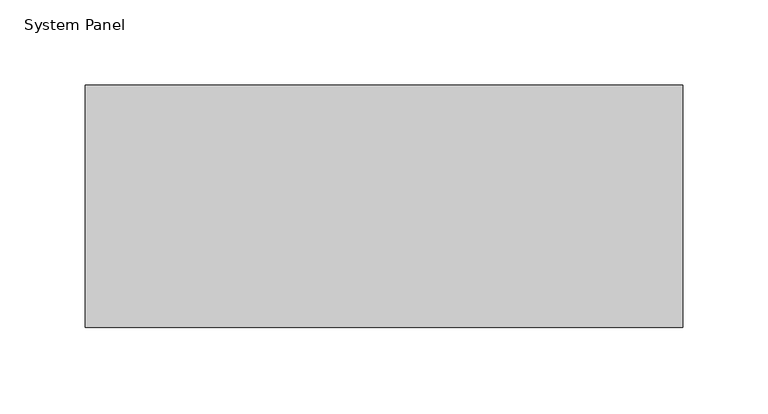
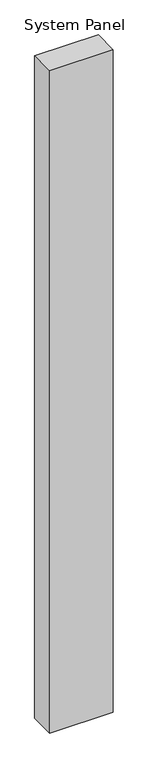
"""IFC4 building model written with IfcOpenShell, lengths in millimetres: plate geometry, System Panel : NLRS_21_CWP_hsb-vulling minerale wol 142 _gen_rsf."""

from ifc_helpers import new_model, si_unit, origin, origin_with_axes, place, context, project, spatial, polyline, outline, extrude, source, transform, mapped, element, save


def system_panel_cc2e8257(model_context):
    return source(origin(), model_context, "Body", "SweptSolid", [
        extrude(outline(polyline([(175.0000002, -71.0), (-175.0000002, -71.0), (-175.0000002, 71.0), (175.0000002, 71.0), (175.0000002, -71.0)])), origin_with_axes(), (0.0, 0.0, 1.0), 3849.0),
    ])


if __name__ == "__main__":
    model = new_model("IFC4")
    model_context = context("Model", 3, world=origin())
    ifc_project = project(units=[si_unit("LENGTHUNIT", "METRE", prefix="MILLI")], contexts=[model_context])
    site = spatial("IfcSite", under=ifc_project)
    building = spatial("IfcBuilding", under=site)
    placement = place(None, origin())
    system_panel_shape = system_panel_cc2e8257(model_context)
    element("IfcPlate", 1, ObjectType="System Panel : NLRS_21_CWP_hsb-vulling minerale wol 142 _gen_rsf", at=placement, inside=building, context=model_context, shape_type="MappedRepresentation", body=[
        mapped(system_panel_shape, transform((0.0, 0.0, 0.0), x_axis=(1.0, 0.0, 0.0), y_axis=(0.0, 1.0, 0.0), z_axis=(0.0, 0.0, 1.0))),
    ])
    save(model, "model.ifc")

# Revit data of these elements
# Type "System Panel : NLRS_21_CWP_hsb-vulling minerale wol 142 _gen_rsf"
#   Export Type to IFC As = "IfcWall"
#   Type IfcGUID = "07M7mRoiH1CR8m_RSKIwpC"
#   Assembly Code = "21.23"
# Element 1 (IfcPlate, "System Panel : NLRS_21_CWP_hsb-vulling minerale wol 142 _gen_rsf")
#   Materials on its faces: "NLRS_m1_isolatie minerale wol_gen_rsf"
# Materials
#   "NLRS_m1_isolatie minerale wol_gen_rsf": class "M - Anorganische materialen", colour RGB 200 200 140, transparency 0, Keynote = "m1", Manufacturer = "Revit Standards Foundation", URL = "www.revitstandards.org", Description = "isolatie minerale wol", Cost = 0
